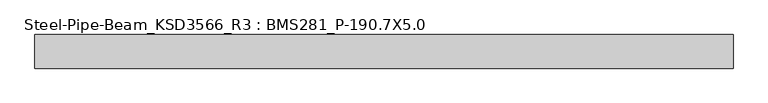
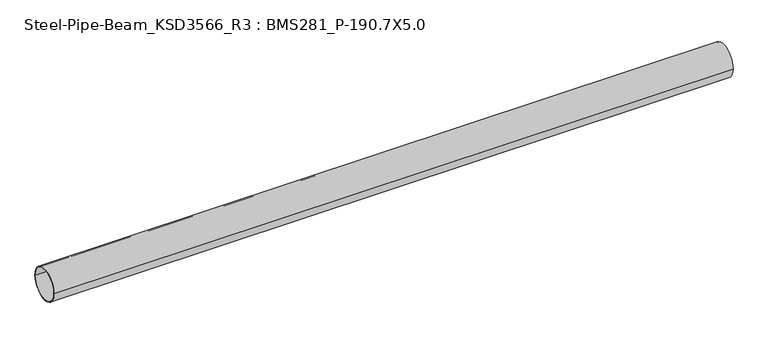
"""IFC4 building model written with IfcOpenShell, lengths in millimetres: member geometry, Steel-Pipe-Beam_KSD3566_R3 : BMS281_P-190.7X5.0."""

from ifc_helpers import new_model, si_unit, point, frame, origin, origin_2d, place, context, project, spatial, circle_curve, trimmed, segment, composite_curve, outline, extrude, source, transform, mapped, element, save


def steel_pipe_beam_ksd3566_r3_bms281_p_190_7x5_0_c6c243b7(model_context):
    return source(origin(), model_context, "Body", "SweptSolid", [
        extrude(outline(composite_curve([segment(trimmed(circle_curve(origin_2d(), 95.35), [point((-95.35, 0.0))], [point((95.35, 0.0))], False, "CARTESIAN"), True, "CONTINUOUS"), segment(trimmed(circle_curve(origin_2d(), 95.35), [point((95.35, 0.0))], [point((-95.35, 0.0))], False, "CARTESIAN"), True, "CONTINUOUS")], self_intersect=False), holes=[composite_curve([segment(trimmed(circle_curve(origin_2d(), 90.35), [point((90.35, 0.0))], [point((-90.35, 0.0))], True, "CARTESIAN"), True, "CONTINUOUS"), segment(trimmed(circle_curve(origin_2d(), 90.35), [point((-90.35, 0.0))], [point((90.35, 0.0))], True, "CARTESIAN"), True, "CONTINUOUS")], self_intersect=False)]), frame((-1975.6500721, 0.0, 0.0), z_axis=(1.0, 0.0, 0.0), x_axis=(0.0, 1.0, 0.0)), (0.0, 0.0, 1.0), 3955.0697928),
    ])


if __name__ == "__main__":
    model = new_model("IFC4")
    model_context = context("Model", 3, world=origin())
    ifc_project = project(units=[si_unit("LENGTHUNIT", "METRE", prefix="MILLI")], contexts=[model_context])
    site = spatial("IfcSite", under=ifc_project)
    building = spatial("IfcBuilding", under=site)
    placement = place(None, origin())
    steel_pipe_beam_ksd3566_r3_bms281_p_190_7x5_0_shape = steel_pipe_beam_ksd3566_r3_bms281_p_190_7x5_0_c6c243b7(model_context)
    element("IfcMember", 1, ObjectType="Steel-Pipe-Beam_KSD3566_R3 : BMS281_P-190.7X5.0", at=placement, inside=building, context=model_context, shape_type="MappedRepresentation", body=[
        mapped(steel_pipe_beam_ksd3566_r3_bms281_p_190_7x5_0_shape, transform((0.0, 0.0, 0.0), x_axis=(1.0, 0.0, 0.0), y_axis=(0.0, 1.0, 0.0), z_axis=(0.0, 0.0, 1.0))),
    ])
    save(model, "model.ifc")

# Revit data of these elements
# Type "Steel-Pipe-Beam_KSD3566_R3 : BMS281_P-190.7X5.0"
#   Keynote = "P-190.7X5.0"
#   SteelWeight = "Light"
#   t = 0.0050 m
#   Surface Area = 0.599102 m²/m
#   Section Area = 29.1697 cm²
#   Mass per Unit Length = 22.8982 kg/m
#   Length [instance default] = 1.5000 m
#   D = 0.1907 m
#   hec_material4 [instance default] = none
#   hec_material3 [instance default] = none
#   hec_material2 [instance default] = none
#   hec_material1 [instance default] = none
#   Structural Material [instance default] = Steel, 45-345
#   Assembly Code = ""
# Element 1 (IfcMember, "Steel-Pipe-Beam_KSD3566_R3 : BMS281_P-190.7X5.0")
#   Structural Material = none
# Materials
#   "Steel, 45-345": class "Metal", colour RGB 189 187 185, transparency 0, Description = "Steel 345 MPa", Cost = 0
